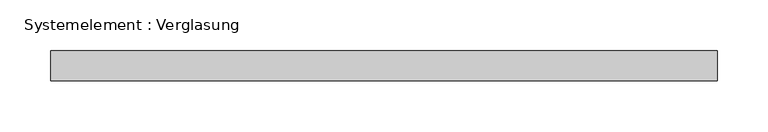
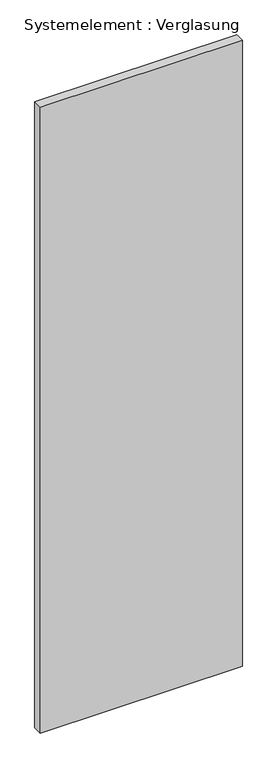
"""IFC4 building model written with IfcOpenShell, lengths in millimetres: plate geometry, Systemelement : Verglasung."""

from ifc_helpers import new_model, si_unit, origin, origin_with_axes, place, context, project, spatial, polyline, outline, extrude, source, transform, mapped, element, save


def systemelement_verglasung_92099b16(model_context):
    return source(origin(), model_context, "Body", "SweptSolid", [
        extrude(outline(polyline([(330.143661, -15.0), (-330.143661, -15.0), (-330.143661, 15.0), (330.143661, 15.0), (330.143661, -15.0)])), origin_with_axes(), (0.0, 0.0, 1.0), 2160.0),
    ])


if __name__ == "__main__":
    model = new_model("IFC4")
    model_context = context("Model", 3, world=origin())
    ifc_project = project(units=[si_unit("LENGTHUNIT", "METRE", prefix="MILLI")], contexts=[model_context])
    site = spatial("IfcSite", under=ifc_project)
    building = spatial("IfcBuilding", under=site)
    placement = place(None, origin())
    systemelement_verglasung_shape = systemelement_verglasung_92099b16(model_context)
    element("IfcPlate", 1, ObjectType="Systemelement : Verglasung", at=placement, inside=building, context=model_context, shape_type="MappedRepresentation", body=[
        mapped(systemelement_verglasung_shape, transform((0.0, 0.0, 0.0), x_axis=(1.0, 0.0, 0.0), y_axis=(0.0, 1.0, 0.0), z_axis=(0.0, 0.0, 1.0))),
    ])
    save(model, "model.ifc")

# Revit data of these elements
# Type "Systemelement : Verglasung"
#   Construction Type Id = "GSP4R"
#   Analytic Construction = "1/8 Zoll Pilkington-Verglasung einfach"
#   Visual Light Transmittance = 0.9
#   Solar Heat Gain Coefficient = 0.86
#   Heat Transfer Coefficient (U) = 6.7069 W/(m²·K)
# Element 1 (IfcPlate, "Systemelement : Verglasung")
#   Materials on its faces: "Glas"
# Materials
#   "Glas": class "Glas", colour RGB 0 0 255, transparency 0.75, Comments = "Render-Darstellung nicht aktualisiert ", Cost = 0
